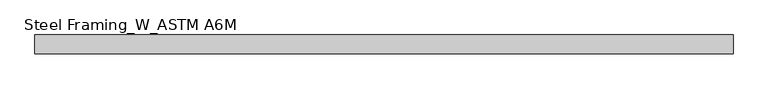
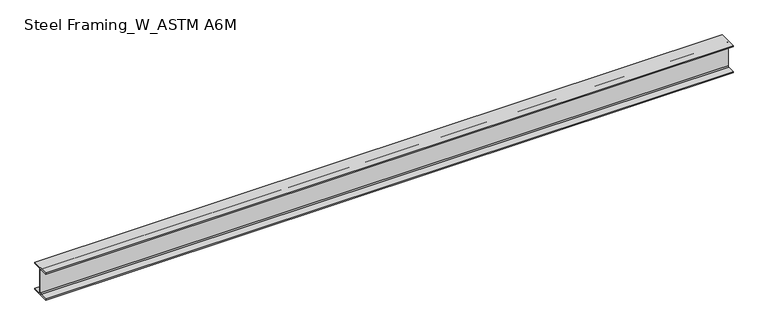
"""IFC4 building model written with IfcOpenShell, lengths in millimetres: beam geometry, Steel Framing_W_ASTM A6M : H_SB_AR_S02_W200x31.3_RB4."""

from ifc_helpers import new_model, si_unit, point, frame, frame_2d, origin, place, context, project, spatial, polyline, circle_curve, trimmed, segment, composite_curve, outline, extrude, source, transform, mapped, element, save


def steel_framing_w_astm_a6m_6c425225(model_context):
    return source(origin(), model_context, "Body", "SweptSolid", [
        extrude(outline(composite_curve([segment(polyline([(67.0, -94.8), (67.0, -105.0), (-67.0, -105.0), (-67.0, -94.8), (-10.775, -94.8)]), True, "CONTINUOUS"), segment(trimmed(circle_curve(frame_2d((-10.775, -87.2)), 7.6), [point((-10.775, -94.8))], [point((-3.175, -87.2))], True, "CARTESIAN"), True, "CONTINUOUS"), segment(polyline([(-3.175, -87.2), (-3.175, 87.2)]), True, "CONTINUOUS"), segment(trimmed(circle_curve(frame_2d((-10.775, 87.2)), 7.6), [point((-3.175, 87.2))], [point((-10.775, 94.8))], True, "CARTESIAN"), True, "CONTINUOUS"), segment(polyline([(-10.775, 94.8), (-67.0, 94.8), (-67.0, 105.0), (67.0, 105.0), (67.0, 94.8), (10.775, 94.8)]), True, "CONTINUOUS"), segment(trimmed(circle_curve(frame_2d((10.775, 87.2)), 7.6), [point((10.775, 94.8))], [point((3.175, 87.2))], True, "CARTESIAN"), True, "CONTINUOUS"), segment(polyline([(3.175, 87.2), (3.175, -87.2)]), True, "CONTINUOUS"), segment(trimmed(circle_curve(frame_2d((10.775, -87.2)), 7.6), [point((3.175, -87.2))], [point((10.775, -94.8))], True, "CARTESIAN"), True, "CONTINUOUS"), segment(polyline([(10.775, -94.8), (67.0, -94.8)]), True, "CONTINUOUS")], self_intersect=False)), frame((-2500.0, 0.0, 0.0), z_axis=(1.0, 0.0, 0.0), x_axis=(0.0, 1.0, 0.0)), (0.0, 0.0, 1.0), 4987.2),
    ])


if __name__ == "__main__":
    model = new_model("IFC4")
    model_context = context("Model", 3, world=origin())
    ifc_project = project(units=[si_unit("LENGTHUNIT", "METRE", prefix="MILLI")], contexts=[model_context])
    site = spatial("IfcSite", under=ifc_project)
    building = spatial("IfcBuilding", under=site)
    placement = place(None, origin())
    steel_framing_w_astm_a6m_shape = steel_framing_w_astm_a6m_6c425225(model_context)
    element("IfcBeam", 1, ObjectType="Steel Framing_W_ASTM A6M : H_SB_AR_S02_W200x31.3_RB4", at=placement, inside=building, context=model_context, shape_type="MappedRepresentation", body=[
        mapped(steel_framing_w_astm_a6m_shape, transform((0.0, 0.0, 0.0), x_axis=(1.0, 0.0, 0.0), y_axis=(0.0, 1.0, 0.0), z_axis=(0.0, 0.0, 1.0))),
    ])
    save(model, "model.ifc")

# Revit data of these elements
# Type "Steel Framing_W_ASTM A6M : H_SB_AR_S02_W200x31.3_RB4"
#   Type Mark = "RB4"
#   Section Name Key = "W8x21"
#   Width = 13.4 cm
#   Web Thickness = 0.635 cm
#   Web Fillet = 0.76 cm
#   Warping Constant = 40800.0 cm⁶
#   Torsional Moment of Inertia = 11.70 cm⁴
#   Section Area = 39.7 cm²
#   Plastic Modulus weak axis = 93.2 cm³
#   Plastic Modulus strong axis = 334.0 cm³
#   Perimeter = 0.93 m²/m
#   Nominal Weight = 31.30 kgf/m
#   Moment of Inertia weak axis = 407.00 cm⁴
#   Moment of Inertia strong axis = 3130.00 cm⁴
#   Height = 21.0 cm
#   Flange Thickness = 1.02 cm
#   Elastic Modulus weak axis = 60.8 cm³
#   Elastic Modulus strong axis = 298.0 cm³
#   Centroid Vertical = 10.5 cm
#   Centroid Horizontal = 6.7 cm
#   Length [instance default] = 1500 mm
#   Structural Material [instance default] = Steel, 45-345
#   Bolt Spacing = 0
#   Assembly Code = ""
# Element 1 (IfcBeam, "Steel Framing_W_ASTM A6M : H_SB_AR_S02_W200x31.3_RB4")
#   Materials on its faces: "Steel, 45-345"
# Materials
#   "Steel, 45-345": class "Metal", colour RGB 189 187 185, transparency 0, Description = "Steel 345 MPa", Cost = 0
